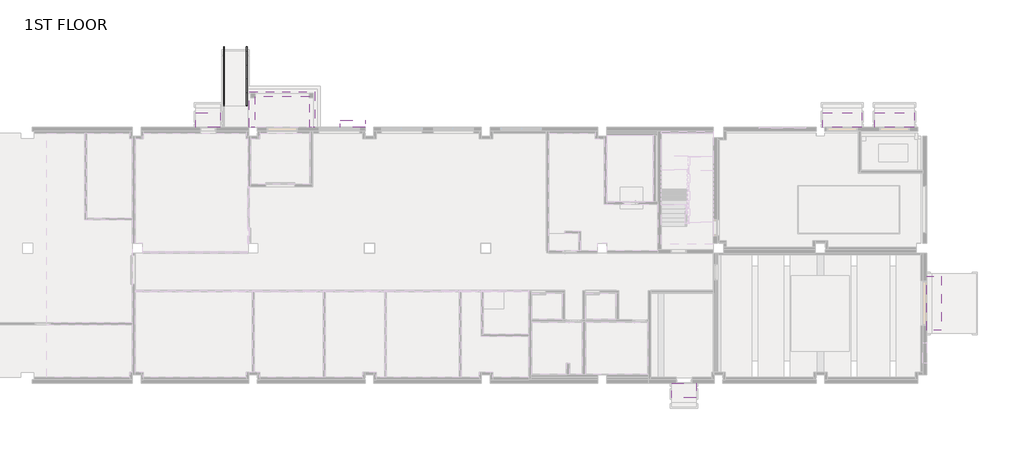
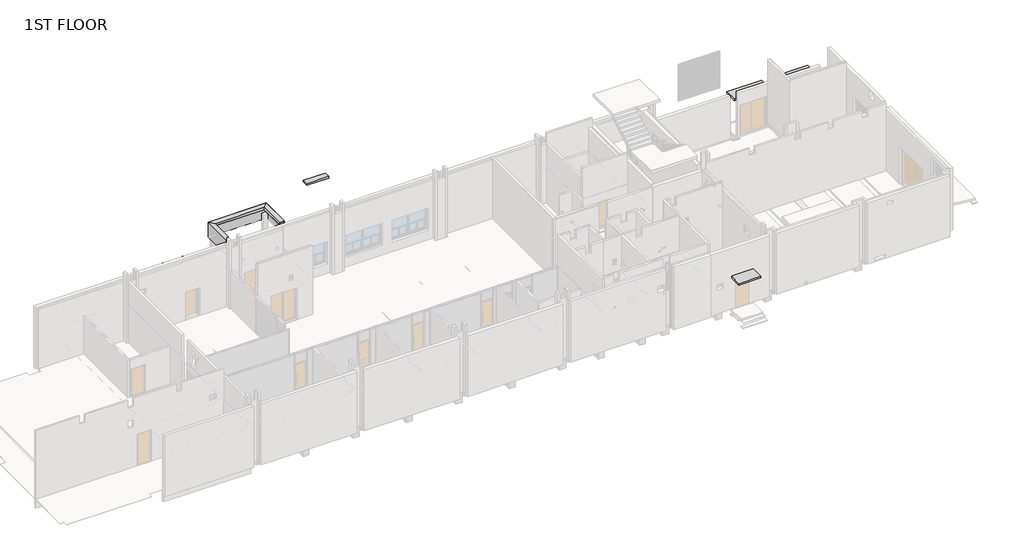
# One storey, part 15 of 15: 7 proxies, 2 railings.
"""IFC4 building model written with IfcOpenShell, lengths in millimetres."""

import ifcopenshell
import ifcopenshell.guid

model = None  # the IFC model being written
_history = None  # IfcOwnerHistory: only IFC2X3 demands one
_inside = {}  # id of a spatial element -> (the spatial element, [elements in it])
_under = {}  # id of a project, library or spatial element -> (it, [spatial elements below it])
_declared = {}  # id of a project -> (the project, [libraries it declares])
_typed = {}  # id of a type object -> (the type object, [elements of that type])
_made_of = {}  # id of a material, layer set ... -> (it, [elements and type objects made of it])


def new_model(schema):
    """Start an empty IFC model of exactly this schema.

    Asked for "IFC4X3", IfcOpenShell would pick the latest addendum, in which some entities
    have other attributes; the version numbers below select the first issue.
    IFC2X3 requires an IfcOwnerHistory on every rooted entity: one is made here for all.
    """
    global model, _history
    if schema == "IFC4X3":
        model = ifcopenshell.file(schema_version=(4, 3, 0, 0))
    else:
        model = ifcopenshell.file(schema=schema)
    _inside.clear()
    _under.clear()
    _declared.clear()
    _typed.clear()
    _made_of.clear()
    _history = None
    if model.schema == "IFC2X3":
        org = make("IfcOrganization", Name="unknown")
        user = make(
            "IfcPersonAndOrganization",
            ThePerson=make("IfcPerson", FamilyName="unknown"),
            TheOrganization=org,
        )
        app = make(
            "IfcApplication",
            ApplicationDeveloper=org,
            Version="unknown",
            ApplicationFullName="unknown",
            ApplicationIdentifier="unknown",
        )
        _history = make(
            "IfcOwnerHistory",
            OwningUser=user,
            OwningApplication=app,
            ChangeAction="ADDED",
            CreationDate=0,
        )
    return model


def make(cls, **values):
    """One entity of the class cls with the attributes given. An attribute that is None is left unset."""
    return model.create_entity(
        cls, **{name: value for name, value in values.items() if value is not None}
    )


def rooted(cls, **values):
    """An entity with a GlobalId (a new one), such as an element, a storey or a relation."""
    return make(cls, GlobalId=ifcopenshell.guid.new(), OwnerHistory=_history, **values)


def si_unit(unit_type, name, prefix=None):
    """IfcSIUnit, for example si_unit("LENGTHUNIT", "METRE", prefix="MILLI")."""
    return make("IfcSIUnit", UnitType=unit_type, Prefix=prefix, Name=name)


def assignment(units):
    """IfcUnitAssignment: the units of a project."""
    return None if units is None else make("IfcUnitAssignment", Units=units)


def point(xyz):
    """IfcCartesianPoint."""
    return None if xyz is None else make("IfcCartesianPoint", Coordinates=xyz)


def direction(xyz):
    """IfcDirection."""
    return None if xyz is None else make("IfcDirection", DirectionRatios=xyz)


def frame(location, z_axis=None, x_axis=None):
    """IfcAxis2Placement3D, a coordinate frame: its origin and axes. An axis left out is left unset."""
    return make(
        "IfcAxis2Placement3D",
        Location=point(location),
        Axis=direction(z_axis),
        RefDirection=direction(x_axis),
    )


def origin():
    """The frame at (0, 0, 0) with its axes left unset."""
    return frame((0.0, 0.0, 0.0))


def place(relative_to, where):
    """IfcLocalPlacement: puts the frame where relative to a parent placement (None: the world)."""
    return make(
        "IfcLocalPlacement", PlacementRelTo=relative_to, RelativePlacement=where
    )


def context(
    kind, dimensions, precision=None, world=None, true_north=None, identifier=None
):
    """IfcGeometricRepresentationContext, for example the 3D "Model" context."""
    return make(
        "IfcGeometricRepresentationContext",
        ContextIdentifier=identifier,
        ContextType=kind,
        CoordinateSpaceDimension=dimensions,
        Precision=precision,
        WorldCoordinateSystem=world,
        TrueNorth=true_north,
    )


def project(units=None, contexts=None):
    """IfcProject with its units and contexts."""
    return rooted(
        "IfcProject",
        Name="project",
        RepresentationContexts=contexts,
        UnitsInContext=assignment(units),
    )


def spatial(cls, under=None, at=None, **own):
    """A site, building, storey or space (cls), placed at a placement, below another one or the project."""
    s = rooted(cls, ObjectPlacement=at, **own)
    if under is not None:
        _under.setdefault(under.id(), (under, []))[1].append(s)
    return s


def polyline(points):
    """IfcPolyline through the points."""
    return make("IfcPolyline", Points=[point(p) for p in points])


def ellipse_curve(where, semi_axis1, semi_axis2):
    """IfcEllipse in the frame where."""
    return make(
        "IfcEllipse", Position=where, SemiAxis1=semi_axis1, SemiAxis2=semi_axis2
    )


def outline(outer, holes=None, kind="AREA"):
    """IfcArbitraryClosedProfileDef: a profile drawn as a closed curve; with holes, ...WithVoids."""
    if holes is None:
        return make("IfcArbitraryClosedProfileDef", ProfileType=kind, OuterCurve=outer)
    return make(
        "IfcArbitraryProfileDefWithVoids",
        ProfileType=kind,
        OuterCurve=outer,
        InnerCurves=holes,
    )


def extrude(swept, where, along, depth):
    """IfcExtrudedAreaSolid: the profile swept, set in the frame where, extruded along a direction by depth."""
    return make(
        "IfcExtrudedAreaSolid",
        SweptArea=swept,
        Position=where,
        ExtrudedDirection=direction(along),
        Depth=depth,
    )


def faces_of(points, faces, orient=None, outer=None):
    """IfcFace entities. A face is a list of loops; a loop is a list of indices into points, from 0.

    orient and outer hold one flag for each loop. By default every Orientation is true, the
    first loop of a face is its IfcFaceOuterBound and the others are IfcFaceBound.
    """
    made = []
    for i, loops in enumerate(faces):
        bounds = []
        for j, loop in enumerate(loops):
            is_outer = j == 0 if outer is None else outer[i][j]
            bounds.append(
                make(
                    "IfcFaceOuterBound" if is_outer else "IfcFaceBound",
                    Bound=make("IfcPolyLoop", Polygon=[points[k] for k in loop]),
                    Orientation=True if orient is None else orient[i][j],
                )
            )
        made.append(make("IfcFace", Bounds=bounds))
    return made


def faceted_brep(points, faces, orient=None, outer=None, voids=None):
    """IfcFacetedBrep: a solid bounded by flat faces; with voids (closed shells), ...WithVoids."""
    shared = [point(p) for p in points]
    hull = make("IfcClosedShell", CfsFaces=faces_of(shared, faces, orient, outer))
    if voids is None:
        return make("IfcFacetedBrep", Outer=hull)
    return make(
        "IfcFacetedBrepWithVoids",
        Outer=hull,
        Voids=[
            make(cls, CfsFaces=faces_of(shared, fs, o, b)) for cls, fs, o, b in voids
        ],
    )


def shape(context_of_items, identifier, shape_type, items):
    """IfcShapeRepresentation: the items that make up one representation, for example the "Body"."""
    return make(
        "IfcShapeRepresentation",
        ContextOfItems=context_of_items,
        RepresentationIdentifier=identifier,
        RepresentationType=shape_type,
        Items=items,
    )


def source(mapping_origin, context_of_items, identifier, shape_type, items):
    """IfcRepresentationMap: a shape defined once, which mapped items show again and again."""
    return make(
        "IfcRepresentationMap",
        MappingOrigin=mapping_origin,
        MappedRepresentation=shape(context_of_items, identifier, shape_type, items),
    )


def transform(
    local_origin,
    x_axis=None,
    y_axis=None,
    z_axis=None,
    scale=None,
    scale2=None,
    scale3=None,
    uniform=True,
):
    """IfcCartesianTransformationOperator3D, or its non-uniform kind. x_axis, y_axis, z_axis: its Axis1, 2, 3."""
    if uniform:
        return make(
            "IfcCartesianTransformationOperator3D",
            Axis1=direction(x_axis),
            Axis2=direction(y_axis),
            LocalOrigin=point(local_origin),
            Scale=scale,
            Axis3=direction(z_axis),
        )
    return make(
        "IfcCartesianTransformationOperator3DnonUniform",
        Axis1=direction(x_axis),
        Axis2=direction(y_axis),
        LocalOrigin=point(local_origin),
        Scale=scale,
        Axis3=direction(z_axis),
        Scale2=scale2,
        Scale3=scale3,
    )


def mapped(mapping_source, mapping_target):
    """IfcMappedItem: shows the shape of a source again, moved by a transform."""
    return make(
        "IfcMappedItem", MappingSource=mapping_source, MappingTarget=mapping_target
    )


def made_of(thing, what):
    """Note that an element or type object is made of a material, layer set ...; save() writes the relation."""
    if what is not None:
        _made_of.setdefault(what.id(), (what, []))[1].append(thing)
    return thing


def element(
    cls,
    number,
    at=None,
    inside=None,
    cuts=None,
    type_object=None,
    material=None,
    context=None,
    identifier="Body",
    shape_type=None,
    held_by="IfcProductDefinitionShape",
    body=None,
    shapes=None,
    **own,
):
    """One element of the class cls, such as IfcWall. Its Tag is "e" and its number.

    at: its placement. inside: the storey or other place that contains it. cuts: it is an
    opening in that element (IfcRelVoidsElement). A single representation is given by context,
    identifier, shape_type and body (its items); several are given by shapes. held_by: the class
    of the entity that holds the representations. save() writes the other relations.
    """
    e = rooted(cls, Tag="e%d" % number, ObjectPlacement=at, **own)
    if body is not None:
        shapes = [shape(context, identifier, shape_type, body)]
    if shapes is not None:
        e.Representation = make(held_by, Representations=shapes)
    if inside is not None:
        _inside.setdefault(inside.id(), (inside, []))[1].append(e)
    if cuts is not None:
        rooted(
            "IfcRelVoidsElement", RelatingBuildingElement=cuts, RelatedOpeningElement=e
        )
    if type_object is not None:
        _typed.setdefault(type_object.id(), (type_object, []))[1].append(e)
    return made_of(e, material)


def aggregate(whole, parts):
    """IfcRelAggregates: a whole, such as a stair, and the parts it consists of."""
    return rooted("IfcRelAggregates", RelatingObject=whole, RelatedObjects=parts)


def save(model, path):
    """Write the relations noted so far, then the file.

    IfcRelAggregates (storeys below a building ...), IfcRelContainedInSpatialStructure (elements
    in a storey), IfcRelDefinesByType, IfcRelAssociatesMaterial and IfcRelDeclares: one each for
    every whole, place, type object, material and project.
    """
    for whole, parts in _under.values():
        aggregate(whole, parts)
    for where, things in _inside.values():
        rooted(
            "IfcRelContainedInSpatialStructure",
            RelatedElements=things,
            RelatingStructure=where,
        )
    for kind, things in _typed.values():
        rooted("IfcRelDefinesByType", RelatedObjects=things, RelatingType=kind)
    for what, things in _made_of.values():
        rooted("IfcRelAssociatesMaterial", RelatedObjects=things, RelatingMaterial=what)
    for by, libraries in _declared.values():
        rooted("IfcRelDeclares", RelatingContext=by, RelatedDefinitions=libraries)
    model.write(path)


def plane_surface(at):
    """IfcPlane: the flat surface through the origin of the frame at, square to its z axis."""
    return make("IfcPlane", Position=at)


def cylinder_surface(at, radius):
    """IfcCylindricalSurface: all points at the distance radius from the z axis of the frame at."""
    return make("IfcCylindricalSurface", Position=at, Radius=radius)


def advanced_brep(points, edges, surfaces, faces):
    """IfcAdvancedBrep: a solid bounded by faces that lie on surfaces and meet in shared edges.

    An edge is (start, end): straight between two places in points (the first is 0);
    or (start, end, curve); or (start, end, curve, False) where it runs against its curve.
    A face is (place in surfaces, loops), or (place, loops, False) where it looks against
    its surface's normal. A loop lists edges by number (the first is 1), with a minus sign
    where the edge is run from its end to its start. The first loop is the outer one.
    """
    corners = [point(p) for p in points]
    vertices = [make("IfcVertexPoint", VertexGeometry=c) for c in corners]
    made = []
    for start, end, *more in edges:
        made.append(
            make(
                "IfcEdgeCurve",
                EdgeStart=vertices[start],
                EdgeEnd=vertices[end],
                EdgeGeometry=more[0] if more else make("IfcPolyline", Points=[corners[start], corners[end]]),
                SameSense=more[1] if len(more) > 1 else True,
            )
        )
    hull = []
    for where, loops, *sense in faces:
        bounds = []
        for j, loop in enumerate(loops):
            ring = [make("IfcOrientedEdge", EdgeElement=made[abs(k) - 1], Orientation=k > 0) for k in loop]
            bounds.append(
                make(
                    "IfcFaceOuterBound" if j == 0 else "IfcFaceBound",
                    Bound=make("IfcEdgeLoop", EdgeList=ring),
                    Orientation=True,
                )
            )
        hull.append(make("IfcAdvancedFace", Bounds=bounds, FaceSurface=surfaces[where], SameSense=sense[0] if sense else True))
    return make("IfcAdvancedBrep", Outer=make("IfcClosedShell", CfsFaces=hull))


def canopy_canopy_239b8731(model_context):
    return source(origin(), model_context, "Body", "SweptSolid", [
        extrude(outline(polyline([(150.0, 0.0), (0.0, 0.0), (0.0, 1000.0), (120.0, 1000.0), (150.0, 0.0)])), frame((-850.0, 0.0, 0.0), z_axis=(1.0, 0.0, 0.0), x_axis=(0.0, 1.0, 0.0)), (0.0, 0.0, 1.0), 1700.0),
    ])


def canopy_canopy_1427068a(model_context):
    return source(origin(), model_context, "Body", "SweptSolid", [
        extrude(outline(polyline([(150.0, 0.0), (0.0, 0.0), (0.0, 1000.0), (120.0, 1000.0), (150.0, 0.0)])), frame((-1350.0, 0.0, 0.0), z_axis=(1.0, 0.0, 0.0), x_axis=(0.0, 1.0, 0.0)), (0.0, 0.0, 1.0), 2700.0),
    ])


def canopy_canopy_da837555(model_context):
    return source(origin(), model_context, "Body", "SweptSolid", [
        extrude(outline(polyline([(150.0, 0.0), (0.0, 0.0), (0.0, 1000.0), (120.0, 1000.0), (150.0, 0.0)])), frame((-1850.0, 0.0, 0.0), z_axis=(1.0, 0.0, 0.0), x_axis=(0.0, 1.0, 0.0)), (0.0, 0.0, 1.0), 3700.0),
    ])


def canopy_canopy_9389d072(model_context):
    return source(origin(), model_context, "Body", "SweptSolid", [
        extrude(outline(polyline([(150.0, 0.0), (0.0, 0.0), (0.0, 500.0), (120.0, 500.0), (150.0, 0.0)])), frame((-850.0, 0.0, 0.0), z_axis=(1.0, 0.0, 0.0), x_axis=(0.0, 1.0, 0.0)), (0.0, 0.0, 1.0), 1700.0),
    ])


def entrance_stainless_finish_entrance_stainless_finish_7ec3a08c(model_context):
    return source(origin(), model_context, "Body", "Brep", [
        faceted_brep([(26900.0, 300.0, 9737.5), (27000.0, 300.0, 9737.5), (27000.0, 300.0, 9740.5), (26903.0, 300.0, 9740.5), (26903.0, 300.0, 9917.2461426), (27247.0, 300.0, 9946.7318569), (27247.0, 300.0, 8700.0), (27250.0, 300.0, 8700.0), (27250.0, 300.0, 9950.0), (26900.0, 300.0, 9920.0), (26900.0, 2400.0, 9737.5), (23100.0, 2400.0, 9737.5), (23100.0, 300.0, 9737.5), (23000.0, 300.0, 9737.5), (23000.0, 2500.0, 9737.5), (27000.0, 2500.0, 9737.5), (27000.0, 2500.0, 9740.5), (23000.0, 2500.0, 9740.5), (23000.0, 300.0, 9740.5), (23097.0, 300.0, 9740.5), (23097.0, 2403.0, 9740.5), (26903.0, 2403.0, 9740.5), (26903.0, 2403.0, 9917.2461426), (27247.0, 2747.0, 9946.7318569), (27247.0, 2747.0, 8700.0), (22753.0, 2747.0, 8700.0), (22753.0, 300.0, 8700.0), (22750.0, 300.0, 8700.0), (22750.0, 2750.0, 8700.0), (27250.0, 2750.0, 8700.0), (27250.0, 2750.0, 9950.0), (26900.0, 2400.0, 9920.0), (23097.0, 2403.0, 9917.2461426), (22753.0, 2747.0, 9946.7318569), (22750.0, 2750.0, 9950.0), (23100.0, 2400.0, 9920.0), (23100.0, 300.0, 9920.0), (22750.0, 300.0, 9950.0), (22753.0, 300.0, 9946.7318569), (23097.0, 300.0, 9917.2461426)], [[[0, 1, 2, 3, 4, 5, 6, 7, 8, 9]], [[1, 0, 10, 11, 12, 13, 14, 15]], [[2, 1, 15, 16]], [[3, 2, 16, 17, 18, 19, 20, 21]], [[4, 3, 21, 22]], [[5, 4, 22, 23]], [[6, 5, 23, 24]], [[7, 6, 24, 25, 26, 27, 28, 29]], [[8, 7, 29, 30]], [[9, 8, 30, 31]], [[0, 9, 31, 10]], [[16, 15, 14, 17]], [[22, 21, 20, 32]], [[23, 22, 32, 33]], [[24, 23, 33, 25]], [[30, 29, 28, 34]], [[31, 30, 34, 35]], [[10, 31, 35, 11]], [[12, 36, 37, 27, 26, 38, 39, 19, 18, 13]], [[17, 14, 13, 18]], [[32, 20, 19, 39]], [[33, 32, 39, 38]], [[25, 33, 38, 26]], [[34, 28, 27, 37]], [[35, 34, 37, 36]], [[11, 35, 36, 12]]]),
    ])


model = new_model("IFC4")

# Units and contexts
model_context = context("Model", 3, world=origin())
ifc_project = project(units=[si_unit("LENGTHUNIT", "METRE", prefix="MILLI")], contexts=[model_context])

# Site, building, storey
site = spatial("IfcSite", under=ifc_project)
building = spatial("IfcBuilding", under=site)
storey = spatial("IfcBuildingStorey", under=building, Name="1ST FLOOR", Elevation=4800.0)

# Proxies
placement = place(None, origin())
canopy_canopy_shape = canopy_canopy_239b8731(model_context)
element("IfcBuildingElementProxy", 1, Name="Canopy : Canopy", ObjectType="Canopy : Canopy", at=placement, inside=storey, context=model_context, shape_type="MappedRepresentation", body=[
    mapped(canopy_canopy_shape, transform((19899.9999999, 300.0, 7410.0), x_axis=(-1.0, 0.0, 0.0), y_axis=(0.0, 0.0, 1.0), z_axis=(0.0, 1.0, 0.0))),
])
element("IfcBuildingElementProxy", 2, Name="Canopy : Canopy", ObjectType="Canopy : Canopy", at=placement, inside=storey, context=model_context, shape_type="MappedRepresentation", body=[
    mapped(canopy_canopy_shape, transform((52624.9999999, -17300.0, 7380.0), x_axis=(1.0, 0.0, 0.0), y_axis=(0.0, 0.0, 1.0), z_axis=(0.0, -1.0, 0.0))),
])
canopy_canopy_2_shape = canopy_canopy_1427068a(model_context)
element("IfcBuildingElementProxy", 3, Name="Canopy : Canopy", ObjectType="Canopy : Canopy", at=placement, inside=storey, context=model_context, shape_type="MappedRepresentation", body=[
    mapped(canopy_canopy_2_shape, transform((63500.0, 300.0, 7590.0), x_axis=(-1.0, 0.0, 0.0), y_axis=(0.0, 0.0, 1.0), z_axis=(0.0, 1.0, 0.0))),
])
element("IfcBuildingElementProxy", 4, Name="Canopy : Canopy", ObjectType="Canopy : Canopy", at=placement, inside=storey, context=model_context, shape_type="MappedRepresentation", body=[
    mapped(canopy_canopy_2_shape, transform((67100.0, 300.0, 7590.0), x_axis=(-1.0, 0.0, 0.0), y_axis=(0.0, 0.0, 1.0), z_axis=(0.0, 1.0, 0.0))),
])
canopy_canopy_3_shape = canopy_canopy_da837555(model_context)
element("IfcBuildingElementProxy", 5, Name="Canopy : Canopy", ObjectType="Canopy : Canopy", at=placement, inside=storey, context=model_context, shape_type="MappedRepresentation", body=[
    mapped(canopy_canopy_3_shape, transform((69300.0, -11800.0, 8180.0), x_axis=(0.0, 1.0, 0.0), y_axis=(0.0, 0.0, 1.0), z_axis=(1.0, 0.0, 0.0))),
])
canopy_canopy_4_shape = canopy_canopy_9389d072(model_context)
element("IfcBuildingElementProxy", 6, Name="Canopy : Canopy", ObjectType="Canopy : Canopy", at=placement, inside=storey, context=model_context, shape_type="MappedRepresentation", body=[
    mapped(canopy_canopy_4_shape, transform((29850.0, 300.0, 12250.0), x_axis=(-1.0, 0.0, 0.0), y_axis=(0.0, 0.0, 1.0), z_axis=(0.0, 1.0, 0.0))),
])
entrance_stainless_finish_entrance_stainless_finish_shape = entrance_stainless_finish_entrance_stainless_finish_7ec3a08c(model_context)
element("IfcBuildingElementProxy", 7, Name="Entrance Stainless Finish : Entrance Stainless Finish", ObjectType="Entrance Stainless Finish : Entrance Stainless Finish", at=placement, inside=storey, context=model_context, shape_type="MappedRepresentation", body=[
    mapped(entrance_stainless_finish_entrance_stainless_finish_shape, transform((0.0, 0.0, 0.0), x_axis=(1.0, 0.0, 0.0), y_axis=(0.0, 1.0, 0.0), z_axis=(0.0, 0.0, 1.0))),
])

# Railings
element("IfcRailing", 8, ObjectType="H_RL_AR_S10_Steel Handrail_H850_Ramp", at=placement, inside=storey, context=model_context, shape_type="AdvancedBrep", body=[
    advanced_brep(
    [(21032.0, 1800.0, 5580.9578246), (20994.0, 1800.0, 5580.9578246), (21032.0, 5850.0, 5310.9578246), (20994.0, 5850.0, 5310.9578246)],
    [
        (0, 1, ellipse_curve(frame((21013.0, 1800.0, 5580.9578246), z_axis=(0.0, -1.0, 0.0), x_axis=(0.0, 0.0, 1.0)), 19.0421754, 19.0)),
        (1, 0, ellipse_curve(frame((21013.0, 1800.0, 5580.9578246), z_axis=(0.0, -1.0, 0.0), x_axis=(0.0, 0.0, 1.0)), 19.0421754, 19.0)),
        (2, 3, ellipse_curve(frame((21013.0, 5850.0, 5310.9578246), z_axis=(0.0, 1.0, 0.0), x_axis=(0.0, 0.0, 1.0)), 19.0421754, 19.0)),
        (3, 2, ellipse_curve(frame((21013.0, 5850.0, 5310.9578246), z_axis=(0.0, 1.0, 0.0), x_axis=(0.0, 0.0, 1.0)), 19.0421754, 19.0)),
        (0, 2),
        (3, 1),
    ],
    [
        plane_surface(frame((21013.0, 1800.0, 5600.0), z_axis=(0.0, -1.0, 0.0), x_axis=(0.0, 0.0, 1.0))),
        plane_surface(frame((21013.0, 5850.0, 5330.0), z_axis=(0.0, 1.0, 0.0), x_axis=(0.0, 0.0, 1.0))),
        cylinder_surface(frame((21013.0, 1798.7361388, 5581.042082), z_axis=(0.0, -0.9977851578566089, 0.06651901052377449), x_axis=(-1.0, 0.0, 0.0)), 19.0),
    ],
    [
        (0, [[1, 2]]),
        (1, [[3, 4]]),
        (2, [[-1, 5, -4, 6]]),
        (2, [[-2, -6, -3, -5]]),
    ],
),
    advanced_brep(
    [(20994.0, 1800.0, 5130.9578246), (21032.0, 1800.0, 5130.9578246), (20994.0, 5850.0, 4860.9578246), (21032.0, 5850.0, 4860.9578246)],
    [
        (0, 1, ellipse_curve(frame((21013.0, 1800.0, 5130.9578246), z_axis=(0.0, -1.0, 0.0), x_axis=(0.0, 0.0, 1.0)), 19.0421754, 19.0)),
        (1, 0, ellipse_curve(frame((21013.0, 1800.0, 5130.9578246), z_axis=(0.0, -1.0, 0.0), x_axis=(0.0, 0.0, 1.0)), 19.0421754, 19.0)),
        (2, 3, ellipse_curve(frame((21013.0, 5850.0, 4860.9578246), z_axis=(0.0, 1.0, 0.0), x_axis=(0.0, 0.0, 1.0)), 19.0421754, 19.0)),
        (3, 2, ellipse_curve(frame((21013.0, 5850.0, 4860.9578246), z_axis=(0.0, 1.0, 0.0), x_axis=(0.0, 0.0, 1.0)), 19.0421754, 19.0)),
        (0, 2),
        (3, 1),
    ],
    [
        plane_surface(frame((21013.0, 1800.0, 5150.0), z_axis=(0.0, -1.0, 0.0), x_axis=(0.0, 0.0, 1.0))),
        plane_surface(frame((21013.0, 5850.0, 4880.0), z_axis=(0.0, 1.0, 0.0), x_axis=(0.0, 0.0, 1.0))),
        cylinder_surface(frame((21013.0, 1798.7361388, 5131.042082), z_axis=(0.0, -0.9977851578566089, 0.06651901052377449), x_axis=(1.0, 0.0, 0.0)), 19.0),
    ],
    [
        (0, [[1, 2]]),
        (1, [[3, 4]]),
        (2, [[-1, 5, -4, 6]]),
        (2, [[-2, -6, -3, -5]]),
    ],
),
    advanced_brep(
    [(21034.2, 5530.0, 5313.2489825), (21034.2, 5530.0, 4501.3333333), (20991.8, 5530.0, 4501.3333333), (20991.8, 5530.0, 5313.2489825)],
    [
        (0, 1),
        (1, 2, ellipse_curve(frame((21013.0, 5530.0, 4501.3333333), z_axis=(0.0, 0.06651901052377411, 0.9977851578566089), x_axis=(0.0, -0.9977851578566088, 0.06651901052377385)), 21.2470589, 21.2)),
        (2, 3),
        (3, 0, ellipse_curve(frame((21013.0, 5530.0, 5313.2489825), z_axis=(0.0, -0.06651901052377368, -0.9977851578566089), x_axis=(0.0, -0.9977851578566088, 0.06651901052377429)), 21.2470589, 21.2)),
        (0, 3, ellipse_curve(frame((21013.0, 5530.0, 5313.2489825), z_axis=(0.0, -0.06651901052377368, -0.9977851578566089), x_axis=(0.0, -0.9977851578566088, 0.06651901052377429)), 21.2470589, 21.2)),
        (2, 1, ellipse_curve(frame((21013.0, 5530.0, 4501.3333333), z_axis=(0.0, 0.06651901052377411, 0.9977851578566089), x_axis=(0.0, -0.9977851578566088, 0.06651901052377385)), 21.2470589, 21.2)),
    ],
    [
        cylinder_surface(frame((21013.0, 5530.0, 4401.3333333), z_axis=(0.0, 0.0, 1.0), x_axis=(-1.0, 0.0, 0.0)), 21.2),
        plane_surface(frame((20988.0, 5555.0, 5311.5823158), z_axis=(0.0, 0.06651901052377368, 0.9977851578566089), x_axis=(1.0, 0.0, 0.0))),
        plane_surface(frame((20988.0, 5505.0, 4503.0), z_axis=(0.0, -0.06651901052377411, -0.9977851578566089), x_axis=(1.0, 0.0, 0.0))),
    ],
    [
        (0, [[1, 2, 3, 4]]),
        (0, [[-1, 5, -3, 6]]),
        (1, [[-4, -5]]),
        (2, [[-2, -6]]),
    ],
),
    advanced_brep(
    [(21034.2, 4580.0, 5376.5823158), (21034.2, 4580.0, 4564.6666667), (20991.8, 4580.0, 4564.6666667), (20991.8, 4580.0, 5376.5823158)],
    [
        (0, 1),
        (1, 2, ellipse_curve(frame((21013.0, 4580.0, 4564.6666667), z_axis=(0.0, 0.06651901052377411, 0.9977851578566089), x_axis=(0.0, -0.9977851578566088, 0.06651901052377385)), 21.2470589, 21.2)),
        (2, 3),
        (3, 0, ellipse_curve(frame((21013.0, 4580.0, 5376.5823158), z_axis=(0.0, -0.06651901052377368, -0.9977851578566089), x_axis=(0.0, -0.9977851578566088, 0.06651901052377429)), 21.2470589, 21.2)),
        (0, 3, ellipse_curve(frame((21013.0, 4580.0, 5376.5823158), z_axis=(0.0, -0.06651901052377368, -0.9977851578566089), x_axis=(0.0, -0.9977851578566088, 0.06651901052377429)), 21.2470589, 21.2)),
        (2, 1, ellipse_curve(frame((21013.0, 4580.0, 4564.6666667), z_axis=(0.0, 0.06651901052377411, 0.9977851578566089), x_axis=(0.0, -0.9977851578566088, 0.06651901052377385)), 21.2470589, 21.2)),
    ],
    [
        cylinder_surface(frame((21013.0, 4580.0, 4464.6666667), z_axis=(0.0, 0.0, 1.0), x_axis=(-1.0, 0.0, 0.0)), 21.2),
        plane_surface(frame((20988.0, 4605.0, 5374.9156492), z_axis=(0.0, 0.06651901052377368, 0.9977851578566089), x_axis=(1.0, 0.0, 0.0))),
        plane_surface(frame((20988.0, 4555.0, 4566.3333333), z_axis=(0.0, -0.06651901052377411, -0.9977851578566089), x_axis=(1.0, 0.0, 0.0))),
    ],
    [
        (0, [[1, 2, 3, 4]]),
        (0, [[-1, 5, -3, 6]]),
        (1, [[-4, -5]]),
        (2, [[-2, -6]]),
    ],
),
    advanced_brep(
    [(21034.2, 3630.0, 5439.9156492), (21034.2, 3630.0, 4628.0), (20991.8, 3630.0, 4628.0), (20991.8, 3630.0, 5439.9156492)],
    [
        (0, 1),
        (1, 2, ellipse_curve(frame((21013.0, 3630.0, 4628.0), z_axis=(0.0, 0.06651901052377411, 0.9977851578566089), x_axis=(0.0, -0.9977851578566088, 0.06651901052377385)), 21.2470589, 21.2)),
        (2, 3),
        (3, 0, ellipse_curve(frame((21013.0, 3630.0, 5439.9156492), z_axis=(0.0, -0.06651901052377368, -0.9977851578566089), x_axis=(0.0, -0.9977851578566088, 0.06651901052377429)), 21.2470589, 21.2)),
        (0, 3, ellipse_curve(frame((21013.0, 3630.0, 5439.9156492), z_axis=(0.0, -0.06651901052377368, -0.9977851578566089), x_axis=(0.0, -0.9977851578566088, 0.06651901052377429)), 21.2470589, 21.2)),
        (2, 1, ellipse_curve(frame((21013.0, 3630.0, 4628.0), z_axis=(0.0, 0.06651901052377411, 0.9977851578566089), x_axis=(0.0, -0.9977851578566088, 0.06651901052377385)), 21.2470589, 21.2)),
    ],
    [
        cylinder_surface(frame((21013.0, 3630.0, 4528.0), z_axis=(0.0, 0.0, 1.0), x_axis=(-1.0, 0.0, 0.0)), 21.2),
        plane_surface(frame((20988.0, 3655.0, 5438.2489825), z_axis=(0.0, 0.06651901052377368, 0.9977851578566089), x_axis=(1.0, 0.0, 0.0))),
        plane_surface(frame((20988.0, 3605.0, 4629.6666667), z_axis=(0.0, -0.06651901052377411, -0.9977851578566089), x_axis=(1.0, 0.0, 0.0))),
    ],
    [
        (0, [[1, 2, 3, 4]]),
        (0, [[-1, 5, -3, 6]]),
        (1, [[-4, -5]]),
        (2, [[-2, -6]]),
    ],
),
    advanced_brep(
    [(21034.2, 2680.0, 5503.2489825), (21034.2, 2680.0, 4691.3333333), (20991.8, 2680.0, 4691.3333333), (20991.8, 2680.0, 5503.2489825)],
    [
        (0, 1),
        (1, 2, ellipse_curve(frame((21013.0, 2680.0, 4691.3333333), z_axis=(0.0, 0.06651901052377411, 0.9977851578566089), x_axis=(0.0, -0.9977851578566088, 0.06651901052377385)), 21.2470589, 21.2)),
        (2, 3),
        (3, 0, ellipse_curve(frame((21013.0, 2680.0, 5503.2489825), z_axis=(0.0, -0.06651901052377368, -0.9977851578566089), x_axis=(0.0, -0.9977851578566088, 0.06651901052377429)), 21.2470589, 21.2)),
        (0, 3, ellipse_curve(frame((21013.0, 2680.0, 5503.2489825), z_axis=(0.0, -0.06651901052377368, -0.9977851578566089), x_axis=(0.0, -0.9977851578566088, 0.06651901052377429)), 21.2470589, 21.2)),
        (2, 1, ellipse_curve(frame((21013.0, 2680.0, 4691.3333333), z_axis=(0.0, 0.06651901052377411, 0.9977851578566089), x_axis=(0.0, -0.9977851578566088, 0.06651901052377385)), 21.2470589, 21.2)),
    ],
    [
        cylinder_surface(frame((21013.0, 2680.0, 4591.3333333), z_axis=(0.0, 0.0, 1.0), x_axis=(-1.0, 0.0, 0.0)), 21.2),
        plane_surface(frame((20988.0, 2705.0, 5501.5823158), z_axis=(0.0, 0.06651901052377368, 0.9977851578566089), x_axis=(1.0, 0.0, 0.0))),
        plane_surface(frame((20988.0, 2655.0, 4693.0), z_axis=(0.0, -0.06651901052377411, -0.9977851578566089), x_axis=(1.0, 0.0, 0.0))),
    ],
    [
        (0, [[1, 2, 3, 4]]),
        (0, [[-1, 5, -3, 6]]),
        (1, [[-4, -5]]),
        (2, [[-2, -6]]),
    ],
),
    advanced_brep(
    [(21034.2, 5837.5, 5292.7489825), (21034.2, 5837.5, 4880.8333333), (20991.8, 5837.5, 4880.8333333), (20991.8, 5837.5, 5292.7489825)],
    [
        (0, 1),
        (1, 2, ellipse_curve(frame((21013.0, 5837.5, 4880.8333333), z_axis=(0.0, 0.06651901052377411, 0.9977851578566089), x_axis=(0.0, -0.9977851578566088, 0.06651901052377385)), 21.2470589, 21.2)),
        (2, 3),
        (3, 0, ellipse_curve(frame((21013.0, 5837.5, 5292.7489825), z_axis=(0.0, -0.06651901052377368, -0.9977851578566089), x_axis=(0.0, -0.9977851578566088, 0.06651901052377429)), 21.2470589, 21.2)),
        (0, 3, ellipse_curve(frame((21013.0, 5837.5, 5292.7489825), z_axis=(0.0, -0.06651901052377368, -0.9977851578566089), x_axis=(0.0, -0.9977851578566088, 0.06651901052377429)), 21.2470589, 21.2)),
        (2, 1, ellipse_curve(frame((21013.0, 5837.5, 4880.8333333), z_axis=(0.0, 0.06651901052377411, 0.9977851578566089), x_axis=(0.0, -0.9977851578566088, 0.06651901052377385)), 21.2470589, 21.2)),
    ],
    [
        cylinder_surface(frame((21013.0, 5837.5, 4780.8333333), z_axis=(0.0, 0.0, 1.0), x_axis=(-1.0, 0.0, 0.0)), 21.2),
        plane_surface(frame((20988.0, 5862.5, 5291.0823158), z_axis=(0.0, 0.06651901052377368, 0.9977851578566089), x_axis=(1.0, 0.0, 0.0))),
        plane_surface(frame((20988.0, 5812.5, 4882.5), z_axis=(0.0, -0.06651901052377411, -0.9977851578566089), x_axis=(1.0, 0.0, 0.0))),
    ],
    [
        (0, [[1, 2, 3, 4]]),
        (0, [[-1, 5, -3, 6]]),
        (1, [[-4, -5]]),
        (2, [[-2, -6]]),
    ],
),
    advanced_brep(
    [(21034.2, 1812.5, 5561.0823158), (21034.2, 1812.5, 4749.1666667), (20991.8, 1812.5, 4749.1666667), (20991.8, 1812.5, 5561.0823158)],
    [
        (0, 1),
        (1, 2, ellipse_curve(frame((21013.0, 1812.5, 4749.1666667), z_axis=(0.0, 0.06651901052377411, 0.9977851578566089), x_axis=(0.0, -0.9977851578566088, 0.06651901052377385)), 21.2470589, 21.2)),
        (2, 3),
        (3, 0, ellipse_curve(frame((21013.0, 1812.5, 5561.0823158), z_axis=(0.0, -0.06651901052377368, -0.9977851578566089), x_axis=(0.0, -0.9977851578566088, 0.06651901052377429)), 21.2470589, 21.2)),
        (0, 3, ellipse_curve(frame((21013.0, 1812.5, 5561.0823158), z_axis=(0.0, -0.06651901052377368, -0.9977851578566089), x_axis=(0.0, -0.9977851578566088, 0.06651901052377429)), 21.2470589, 21.2)),
        (2, 1, ellipse_curve(frame((21013.0, 1812.5, 4749.1666667), z_axis=(0.0, 0.06651901052377411, 0.9977851578566089), x_axis=(0.0, -0.9977851578566088, 0.06651901052377385)), 21.2470589, 21.2)),
    ],
    [
        cylinder_surface(frame((21013.0, 1812.5, 4649.1666667), z_axis=(0.0, 0.0, 1.0), x_axis=(-1.0, 0.0, 0.0)), 21.2),
        plane_surface(frame((20988.0, 1837.5, 5559.4156492), z_axis=(0.0, 0.06651901052377368, 0.9977851578566089), x_axis=(1.0, 0.0, 0.0))),
        plane_surface(frame((20988.0, 1787.5, 4750.8333333), z_axis=(0.0, -0.06651901052377411, -0.9977851578566089), x_axis=(1.0, 0.0, 0.0))),
    ],
    [
        (0, [[1, 2, 3, 4]]),
        (0, [[-1, 5, -3, 6]]),
        (1, [[-4, -5]]),
        (2, [[-2, -6]]),
    ],
),
])
element("IfcRailing", 9, ObjectType="H_RL_AR_S10_Steel Handrail_H850_Ramp", at=placement, inside=storey, context=model_context, shape_type="AdvancedBrep", body=[
    advanced_brep(
    [(22582.0, 1800.0, 5580.9578246), (22544.0, 1800.0, 5580.9578246), (22582.0, 5850.0, 5310.9578246), (22544.0, 5850.0, 5310.9578246)],
    [
        (0, 1, ellipse_curve(frame((22563.0, 1800.0, 5580.9578246), z_axis=(0.0, -1.0, 0.0), x_axis=(0.0, 0.0, 1.0)), 19.0421754, 19.0)),
        (1, 0, ellipse_curve(frame((22563.0, 1800.0, 5580.9578246), z_axis=(0.0, -1.0, 0.0), x_axis=(0.0, 0.0, 1.0)), 19.0421754, 19.0)),
        (2, 3, ellipse_curve(frame((22563.0, 5850.0, 5310.9578246), z_axis=(0.0, 1.0, 0.0), x_axis=(0.0, 0.0, 1.0)), 19.0421754, 19.0)),
        (3, 2, ellipse_curve(frame((22563.0, 5850.0, 5310.9578246), z_axis=(0.0, 1.0, 0.0), x_axis=(0.0, 0.0, 1.0)), 19.0421754, 19.0)),
        (0, 2),
        (3, 1),
    ],
    [
        plane_surface(frame((22563.0, 1800.0, 5600.0), z_axis=(0.0, -1.0, 0.0), x_axis=(0.0, 0.0, 1.0))),
        plane_surface(frame((22563.0, 5850.0, 5330.0), z_axis=(0.0, 1.0, 0.0), x_axis=(0.0, 0.0, 1.0))),
        cylinder_surface(frame((22563.0, 1798.7361388, 5581.042082), z_axis=(0.0, -0.9977851578566089, 0.06651901052377422), x_axis=(-1.0, 0.0, 0.0)), 19.0),
    ],
    [
        (0, [[1, 2]]),
        (1, [[3, 4]]),
        (2, [[-1, 5, -4, 6]]),
        (2, [[-2, -6, -3, -5]]),
    ],
),
    advanced_brep(
    [(22544.0, 1800.0, 5130.9578246), (22582.0, 1800.0, 5130.9578246), (22544.0, 5850.0, 4860.9578246), (22582.0, 5850.0, 4860.9578246)],
    [
        (0, 1, ellipse_curve(frame((22563.0, 1800.0, 5130.9578246), z_axis=(0.0, -1.0, 0.0), x_axis=(0.0, 0.0, 1.0)), 19.0421754, 19.0)),
        (1, 0, ellipse_curve(frame((22563.0, 1800.0, 5130.9578246), z_axis=(0.0, -1.0, 0.0), x_axis=(0.0, 0.0, 1.0)), 19.0421754, 19.0)),
        (2, 3, ellipse_curve(frame((22563.0, 5850.0, 4860.9578246), z_axis=(0.0, 1.0, 0.0), x_axis=(0.0, 0.0, 1.0)), 19.0421754, 19.0)),
        (3, 2, ellipse_curve(frame((22563.0, 5850.0, 4860.9578246), z_axis=(0.0, 1.0, 0.0), x_axis=(0.0, 0.0, 1.0)), 19.0421754, 19.0)),
        (0, 2),
        (3, 1),
    ],
    [
        plane_surface(frame((22563.0, 1800.0, 5150.0), z_axis=(0.0, -1.0, 0.0), x_axis=(0.0, 0.0, 1.0))),
        plane_surface(frame((22563.0, 5850.0, 4880.0), z_axis=(0.0, 1.0, 0.0), x_axis=(0.0, 0.0, 1.0))),
        cylinder_surface(frame((22563.0, 1798.7361388, 5131.042082), z_axis=(0.0, -0.9977851578566089, 0.06651901052377422), x_axis=(1.0, 0.0, 0.0)), 19.0),
    ],
    [
        (0, [[1, 2]]),
        (1, [[3, 4]]),
        (2, [[-1, 5, -4, 6]]),
        (2, [[-2, -6, -3, -5]]),
    ],
),
    advanced_brep(
    [(22584.2, 5530.0, 5313.2489825), (22584.2, 5530.0, 4501.3333333), (22541.8, 5530.0, 4501.3333333), (22541.8, 5530.0, 5313.2489825)],
    [
        (0, 1),
        (1, 2, ellipse_curve(frame((22563.0, 5530.0, 4501.3333333), z_axis=(0.0, 0.06651901052377411, 0.9977851578566089), x_axis=(0.0, -0.9977851578566088, 0.06651901052377385)), 21.2470589, 21.2)),
        (2, 3),
        (3, 0, ellipse_curve(frame((22563.0, 5530.0, 5313.2489825), z_axis=(0.0, -0.06651901052377368, -0.9977851578566089), x_axis=(0.0, -0.9977851578566088, 0.06651901052377429)), 21.2470589, 21.2)),
        (0, 3, ellipse_curve(frame((22563.0, 5530.0, 5313.2489825), z_axis=(0.0, -0.06651901052377368, -0.9977851578566089), x_axis=(0.0, -0.9977851578566088, 0.06651901052377429)), 21.2470589, 21.2)),
        (2, 1, ellipse_curve(frame((22563.0, 5530.0, 4501.3333333), z_axis=(0.0, 0.06651901052377411, 0.9977851578566089), x_axis=(0.0, -0.9977851578566088, 0.06651901052377385)), 21.2470589, 21.2)),
    ],
    [
        cylinder_surface(frame((22563.0, 5530.0, 4401.3333333), z_axis=(0.0, 0.0, 1.0), x_axis=(-1.0, 0.0, 0.0)), 21.2),
        plane_surface(frame((22538.0, 5555.0, 5311.5823158), z_axis=(0.0, 0.06651901052377368, 0.9977851578566089), x_axis=(1.0, 0.0, 0.0))),
        plane_surface(frame((22538.0, 5505.0, 4503.0), z_axis=(0.0, -0.06651901052377411, -0.9977851578566089), x_axis=(1.0, 0.0, 0.0))),
    ],
    [
        (0, [[1, 2, 3, 4]]),
        (0, [[-1, 5, -3, 6]]),
        (1, [[-4, -5]]),
        (2, [[-2, -6]]),
    ],
),
    advanced_brep(
    [(22584.2, 4580.0, 5376.5823158), (22584.2, 4580.0, 4564.6666667), (22541.8, 4580.0, 4564.6666667), (22541.8, 4580.0, 5376.5823158)],
    [
        (0, 1),
        (1, 2, ellipse_curve(frame((22563.0, 4580.0, 4564.6666667), z_axis=(0.0, 0.06651901052377411, 0.9977851578566089), x_axis=(0.0, -0.9977851578566088, 0.06651901052377385)), 21.2470589, 21.2)),
        (2, 3),
        (3, 0, ellipse_curve(frame((22563.0, 4580.0, 5376.5823158), z_axis=(0.0, -0.06651901052377368, -0.9977851578566089), x_axis=(0.0, -0.9977851578566088, 0.06651901052377429)), 21.2470589, 21.2)),
        (0, 3, ellipse_curve(frame((22563.0, 4580.0, 5376.5823158), z_axis=(0.0, -0.06651901052377368, -0.9977851578566089), x_axis=(0.0, -0.9977851578566088, 0.06651901052377429)), 21.2470589, 21.2)),
        (2, 1, ellipse_curve(frame((22563.0, 4580.0, 4564.6666667), z_axis=(0.0, 0.06651901052377411, 0.9977851578566089), x_axis=(0.0, -0.9977851578566088, 0.06651901052377385)), 21.2470589, 21.2)),
    ],
    [
        cylinder_surface(frame((22563.0, 4580.0, 4464.6666667), z_axis=(0.0, 0.0, 1.0), x_axis=(-1.0, 0.0, 0.0)), 21.2),
        plane_surface(frame((22538.0, 4605.0, 5374.9156492), z_axis=(0.0, 0.06651901052377368, 0.9977851578566089), x_axis=(1.0, 0.0, 0.0))),
        plane_surface(frame((22538.0, 4555.0, 4566.3333333), z_axis=(0.0, -0.06651901052377411, -0.9977851578566089), x_axis=(1.0, 0.0, 0.0))),
    ],
    [
        (0, [[1, 2, 3, 4]]),
        (0, [[-1, 5, -3, 6]]),
        (1, [[-4, -5]]),
        (2, [[-2, -6]]),
    ],
),
    advanced_brep(
    [(22584.2, 3630.0, 5439.9156492), (22584.2, 3630.0, 4628.0), (22541.8, 3630.0, 4628.0), (22541.8, 3630.0, 5439.9156492)],
    [
        (0, 1),
        (1, 2, ellipse_curve(frame((22563.0, 3630.0, 4628.0), z_axis=(0.0, 0.06651901052377411, 0.9977851578566089), x_axis=(0.0, -0.9977851578566088, 0.06651901052377385)), 21.2470589, 21.2)),
        (2, 3),
        (3, 0, ellipse_curve(frame((22563.0, 3630.0, 5439.9156492), z_axis=(0.0, -0.06651901052377368, -0.9977851578566089), x_axis=(0.0, -0.9977851578566088, 0.06651901052377429)), 21.2470589, 21.2)),
        (0, 3, ellipse_curve(frame((22563.0, 3630.0, 5439.9156492), z_axis=(0.0, -0.06651901052377368, -0.9977851578566089), x_axis=(0.0, -0.9977851578566088, 0.06651901052377429)), 21.2470589, 21.2)),
        (2, 1, ellipse_curve(frame((22563.0, 3630.0, 4628.0), z_axis=(0.0, 0.06651901052377411, 0.9977851578566089), x_axis=(0.0, -0.9977851578566088, 0.06651901052377385)), 21.2470589, 21.2)),
    ],
    [
        cylinder_surface(frame((22563.0, 3630.0, 4528.0), z_axis=(0.0, 0.0, 1.0), x_axis=(-1.0, 0.0, 0.0)), 21.2),
        plane_surface(frame((22538.0, 3655.0, 5438.2489825), z_axis=(0.0, 0.06651901052377368, 0.9977851578566089), x_axis=(1.0, 0.0, 0.0))),
        plane_surface(frame((22538.0, 3605.0, 4629.6666667), z_axis=(0.0, -0.06651901052377411, -0.9977851578566089), x_axis=(1.0, 0.0, 0.0))),
    ],
    [
        (0, [[1, 2, 3, 4]]),
        (0, [[-1, 5, -3, 6]]),
        (1, [[-4, -5]]),
        (2, [[-2, -6]]),
    ],
),
    advanced_brep(
    [(22584.2, 2680.0, 5503.2489825), (22584.2, 2680.0, 4691.3333333), (22541.8, 2680.0, 4691.3333333), (22541.8, 2680.0, 5503.2489825)],
    [
        (0, 1),
        (1, 2, ellipse_curve(frame((22563.0, 2680.0, 4691.3333333), z_axis=(0.0, 0.06651901052377411, 0.9977851578566089), x_axis=(0.0, -0.9977851578566088, 0.06651901052377385)), 21.2470589, 21.2)),
        (2, 3),
        (3, 0, ellipse_curve(frame((22563.0, 2680.0, 5503.2489825), z_axis=(0.0, -0.06651901052377368, -0.9977851578566089), x_axis=(0.0, -0.9977851578566088, 0.06651901052377429)), 21.2470589, 21.2)),
        (0, 3, ellipse_curve(frame((22563.0, 2680.0, 5503.2489825), z_axis=(0.0, -0.06651901052377368, -0.9977851578566089), x_axis=(0.0, -0.9977851578566088, 0.06651901052377429)), 21.2470589, 21.2)),
        (2, 1, ellipse_curve(frame((22563.0, 2680.0, 4691.3333333), z_axis=(0.0, 0.06651901052377411, 0.9977851578566089), x_axis=(0.0, -0.9977851578566088, 0.06651901052377385)), 21.2470589, 21.2)),
    ],
    [
        cylinder_surface(frame((22563.0, 2680.0, 4591.3333333), z_axis=(0.0, 0.0, 1.0), x_axis=(-1.0, 0.0, 0.0)), 21.2),
        plane_surface(frame((22538.0, 2705.0, 5501.5823158), z_axis=(0.0, 0.06651901052377368, 0.9977851578566089), x_axis=(1.0, 0.0, 0.0))),
        plane_surface(frame((22538.0, 2655.0, 4693.0), z_axis=(0.0, -0.06651901052377411, -0.9977851578566089), x_axis=(1.0, 0.0, 0.0))),
    ],
    [
        (0, [[1, 2, 3, 4]]),
        (0, [[-1, 5, -3, 6]]),
        (1, [[-4, -5]]),
        (2, [[-2, -6]]),
    ],
),
    advanced_brep(
    [(22584.2, 5837.5, 5292.7489825), (22584.2, 5837.5, 4880.8333333), (22541.8, 5837.5, 4880.8333333), (22541.8, 5837.5, 5292.7489825)],
    [
        (0, 1),
        (1, 2, ellipse_curve(frame((22563.0, 5837.5, 4880.8333333), z_axis=(0.0, 0.06651901052377411, 0.9977851578566089), x_axis=(0.0, -0.9977851578566088, 0.06651901052377385)), 21.2470589, 21.2)),
        (2, 3),
        (3, 0, ellipse_curve(frame((22563.0, 5837.5, 5292.7489825), z_axis=(0.0, -0.06651901052377368, -0.9977851578566089), x_axis=(0.0, -0.9977851578566088, 0.06651901052377429)), 21.2470589, 21.2)),
        (0, 3, ellipse_curve(frame((22563.0, 5837.5, 5292.7489825), z_axis=(0.0, -0.06651901052377368, -0.9977851578566089), x_axis=(0.0, -0.9977851578566088, 0.06651901052377429)), 21.2470589, 21.2)),
        (2, 1, ellipse_curve(frame((22563.0, 5837.5, 4880.8333333), z_axis=(0.0, 0.06651901052377411, 0.9977851578566089), x_axis=(0.0, -0.9977851578566088, 0.06651901052377385)), 21.2470589, 21.2)),
    ],
    [
        cylinder_surface(frame((22563.0, 5837.5, 4780.8333333), z_axis=(0.0, 0.0, 1.0), x_axis=(-1.0, 0.0, 0.0)), 21.2),
        plane_surface(frame((22538.0, 5862.5, 5291.0823158), z_axis=(0.0, 0.06651901052377368, 0.9977851578566089), x_axis=(1.0, 0.0, 0.0))),
        plane_surface(frame((22538.0, 5812.5, 4882.5), z_axis=(0.0, -0.06651901052377411, -0.9977851578566089), x_axis=(1.0, 0.0, 0.0))),
    ],
    [
        (0, [[1, 2, 3, 4]]),
        (0, [[-1, 5, -3, 6]]),
        (1, [[-4, -5]]),
        (2, [[-2, -6]]),
    ],
),
    advanced_brep(
    [(22584.2, 1812.5, 5561.0823158), (22584.2, 1812.5, 4749.1666667), (22541.8, 1812.5, 4749.1666667), (22541.8, 1812.5, 5561.0823158)],
    [
        (0, 1),
        (1, 2, ellipse_curve(frame((22563.0, 1812.5, 4749.1666667), z_axis=(0.0, 0.06651901052377411, 0.9977851578566089), x_axis=(0.0, -0.9977851578566088, 0.06651901052377385)), 21.2470589, 21.2)),
        (2, 3),
        (3, 0, ellipse_curve(frame((22563.0, 1812.5, 5561.0823158), z_axis=(0.0, -0.06651901052377368, -0.9977851578566089), x_axis=(0.0, -0.9977851578566088, 0.06651901052377429)), 21.2470589, 21.2)),
        (0, 3, ellipse_curve(frame((22563.0, 1812.5, 5561.0823158), z_axis=(0.0, -0.06651901052377368, -0.9977851578566089), x_axis=(0.0, -0.9977851578566088, 0.06651901052377429)), 21.2470589, 21.2)),
        (2, 1, ellipse_curve(frame((22563.0, 1812.5, 4749.1666667), z_axis=(0.0, 0.06651901052377411, 0.9977851578566089), x_axis=(0.0, -0.9977851578566088, 0.06651901052377385)), 21.2470589, 21.2)),
    ],
    [
        cylinder_surface(frame((22563.0, 1812.5, 4649.1666667), z_axis=(0.0, 0.0, 1.0), x_axis=(-1.0, 0.0, 0.0)), 21.2),
        plane_surface(frame((22538.0, 1837.5, 5559.4156492), z_axis=(0.0, 0.06651901052377368, 0.9977851578566089), x_axis=(1.0, 0.0, 0.0))),
        plane_surface(frame((22538.0, 1787.5, 4750.8333333), z_axis=(0.0, -0.06651901052377411, -0.9977851578566089), x_axis=(1.0, 0.0, 0.0))),
    ],
    [
        (0, [[1, 2, 3, 4]]),
        (0, [[-1, 5, -3, 6]]),
        (1, [[-4, -5]]),
        (2, [[-2, -6]]),
    ],
),
])

save(model, "model.ifc")

# Revit data of these elements
# Type "Canopy : Canopy"
#   Type Comments = "CV-AG"
#   H_Rebar Ratio = 0.1
#   Canopy Width [instance default] = 1700 mm
#   Canopy Length [instance default] = 1000 mm
#   Canopy L.P = 120 mm
#   Canopy H.P = 150 mm
#   구조재료 = Concrete_f'c=28MPa(Cylender)
#   Default Elevation = 0
# Type "H_RL_AR_S10_Steel Handrail_H850_Ramp"
#   built-in parameter 1008612 = 0.166667 (stored number, unit not read)
#   built-in parameter 1008611 = 0.166667 (stored number, unit not read)
#   built-in parameter 1008609 = 0.459318 (stored number, unit not read)
#   built-in parameter 1008604 = 0.25 (stored number, unit not read)
#   built-in parameter 1008603 = 0.166667 (stored number, unit not read)
#   Railing Height = 850 mm
#   built-in parameter 1008610 = 1
#   built-in parameter 1008618 = M_Baluster - Square : 25mm
# Elements 1, 2 (IfcBuildingElementProxy, "Canopy : Canopy")
#   Canopy Width = 1700 mm
#   Canopy Length = 1000 mm
#   Phase Created = New Construction
#   Materials on its faces: "Concrete_f'c=28MPa(Cylender)"
# Elements 3, 4 (IfcBuildingElementProxy, "Canopy : Canopy")
#   Canopy Width = 2700 mm
#   Canopy Length = 1000 mm
#   Phase Created = New Construction
#   Materials on its faces: "Concrete_f'c=28MPa(Cylender)"
# Element 5 (IfcBuildingElementProxy, "Canopy : Canopy")
#   Canopy Width = 3700 mm
#   Canopy Length = 1000 mm
#   Phase Created = New Construction
#   Materials on its faces: "Concrete_f'c=28MPa(Cylender)"
# Element 6 (IfcBuildingElementProxy, "Canopy : Canopy")
#   Canopy Width = 1700 mm
#   Canopy Length = 500 mm
#   Phase Created = New Construction
#   Materials on its faces: "Concrete_f'c=28MPa(Cylender)"
# Element 7 (IfcBuildingElementProxy, "Entrance Stainless Finish : Entrance Stainless Finish")
#   Phase Created = New Construction
#   Materials on its faces: "00.Finish_Stainless Hairline"
# Elements 8, 9 (IfcRailing, "H_RL_AR_S10_Steel Handrail_H850_Ramp")
#   Phase Created = New Construction
# Materials
#   "Concrete_f'c=28MPa(Cylender)": class "Concrete", colour RGB 176 176 176, transparency 0, Description = "Reinf. Conc.", Cost = 0, Image = Concrete.Cast-In-Place.Flat.Polished.Grey.jpg
#   "00.Finish_Stainless Hairline": class "Generic", colour RGB 149 149 149, transparency 0, Description = "Acoustic ceiling tile", Cost = 0
